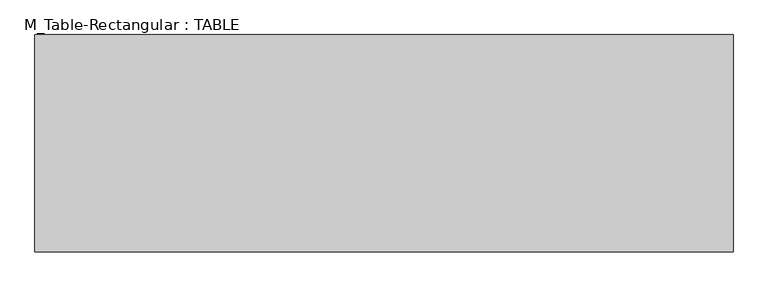
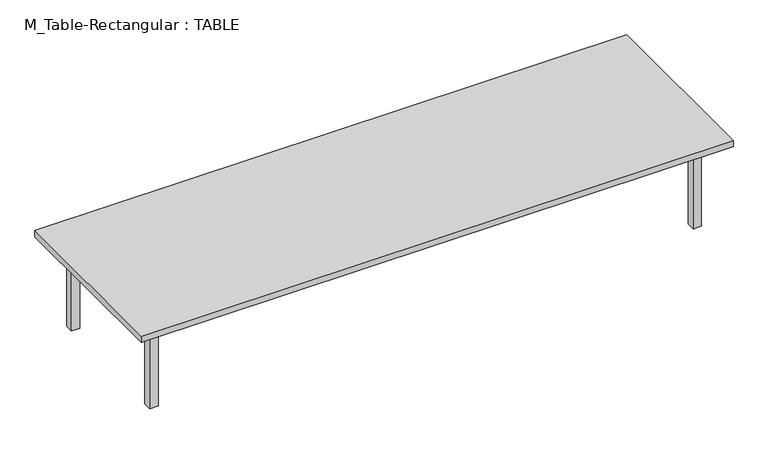
"""IFC4 building model written with IfcOpenShell, lengths in millimetres: furniture geometry, M_Table-Rectangular : TABLE."""

from ifc_helpers import new_model, si_unit, frame, origin, origin_with_axes, place, context, project, spatial, polyline, outline, extrude, source, transform, mapped, element, save


def m_table_rectangular_table_5a2d8c47(model_context):
    return source(origin(), model_context, "Body", "SweptSolid", [
        extrude(outline(polyline([(-2034.1, 547.6), (-2034.1, 484.1), (-2097.6, 484.1), (-2097.6, 547.6), (-2034.1, 547.6)])), origin_with_axes(), (0.0, 0.0, 1.0), 679.2),
        extrude(outline(polyline([(2034.1, 547.6), (2097.6, 547.6), (2097.6, 484.1), (2034.1, 484.1), (2034.1, 547.6)])), origin_with_axes(), (0.0, 0.0, 1.0), 679.2),
        extrude(outline(polyline([(-2034.1, -547.6), (-2097.6, -547.6), (-2097.6, -484.1), (-2034.1, -484.1), (-2034.1, -547.6)])), origin_with_axes(), (0.0, 0.0, 1.0), 679.2),
        extrude(outline(polyline([(2034.1, -547.6), (2034.1, -484.1), (2097.6, -484.1), (2097.6, -547.6), (2034.1, -547.6)])), origin_with_axes(), (0.0, 0.0, 1.0), 679.2),
        extrude(outline(polyline([(2250.0, 700.0), (2250.0, -700.0), (-2250.0, -700.0), (-2250.0, 700.0), (2250.0, 700.0)])), frame((0.0, 0.0, 679.2), z_axis=(0.0, 0.0, 1.0), x_axis=(1.0, 0.0, 0.0)), (0.0, 0.0, 1.0), 50.8),
        extrude(outline(polyline([(2034.1, 509.5), (2034.1, 484.1), (-2034.1, 484.1), (-2034.1, 509.5), (2034.1, 509.5)])), frame((0.0, 0.0, 577.6), z_axis=(0.0, 0.0, 1.0), x_axis=(1.0, 0.0, 0.0)), (0.0, 0.0, 1.0), 101.6),
        extrude(outline(polyline([(2034.1, -509.5), (-2034.1, -509.5), (-2034.1, -484.1), (2034.1, -484.1), (2034.1, -509.5)])), frame((0.0, 0.0, 577.6), z_axis=(0.0, 0.0, 1.0), x_axis=(1.0, 0.0, 0.0)), (0.0, 0.0, 1.0), 101.6),
        extrude(outline(polyline([(-2046.8, -484.1), (-2072.2, -484.1), (-2072.2, 484.1), (-2046.8, 484.1), (-2046.8, -484.1)])), frame((0.0, 0.0, 577.6), z_axis=(0.0, 0.0, 1.0), x_axis=(1.0, 0.0, 0.0)), (0.0, 0.0, 1.0), 101.6),
        extrude(outline(polyline([(2046.8, -484.1), (2046.8, 484.1), (2072.2, 484.1), (2072.2, -484.1), (2046.8, -484.1)])), frame((0.0, 0.0, 577.6), z_axis=(0.0, 0.0, 1.0), x_axis=(1.0, 0.0, 0.0)), (0.0, 0.0, 1.0), 101.6),
    ])


if __name__ == "__main__":
    model = new_model("IFC4")
    model_context = context("Model", 3, world=origin())
    ifc_project = project(units=[si_unit("LENGTHUNIT", "METRE", prefix="MILLI")], contexts=[model_context])
    site = spatial("IfcSite", under=ifc_project)
    building = spatial("IfcBuilding", under=site)
    placement = place(None, origin())
    m_table_rectangular_table_shape = m_table_rectangular_table_5a2d8c47(model_context)
    element("IfcFurniture", 1, ObjectType="M_Table-Rectangular : TABLE", at=placement, inside=building, context=model_context, shape_type="MappedRepresentation", body=[
        mapped(m_table_rectangular_table_shape, transform((0.0, 0.0, 0.0), x_axis=(1.0, 0.0, 0.0), y_axis=(0.0, 1.0, 0.0), z_axis=(0.0, 0.0, 1.0))),
    ])
    save(model, "model.ifc")

# Revit data of these elements
# Type "M_Table-Rectangular : TABLE"
#   Height = 730 mm
#   Length = 4500 mm
#   Width = 1400 mm
#   Base Material = Birch
#   Top Material = Birch
#   Default Elevation = 0
# Element 1 (IfcFurniture, "M_Table-Rectangular : TABLE")
#   Materials on its faces: "Birch"
# Materials
#   "Birch": class "Wood", colour RGB 224 178 126, transparency 0, Description = "Betula Alleghaniensis", Cost = 0
